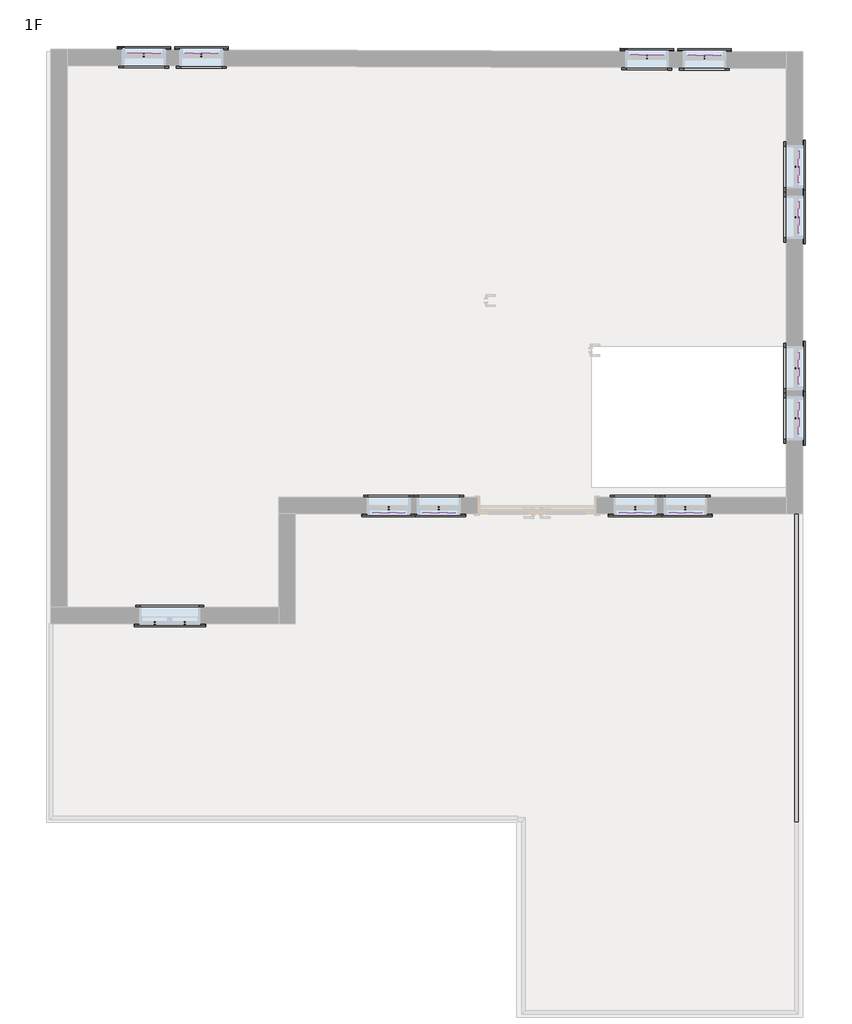
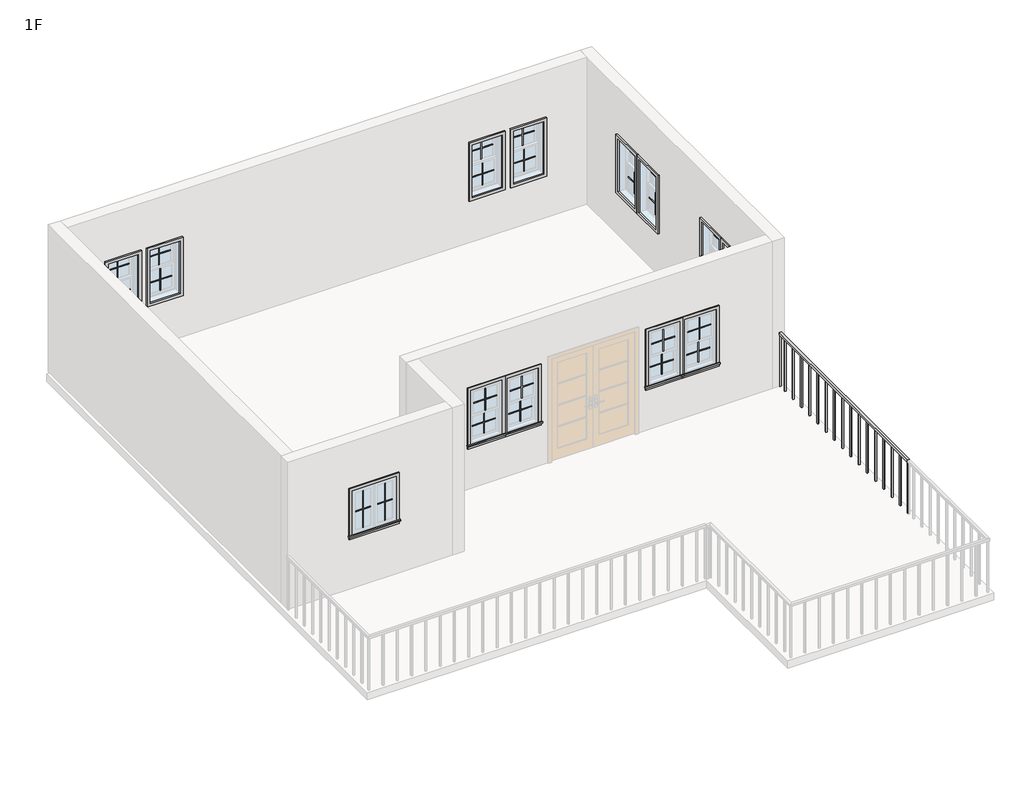
# One storey, part 2 of 2: 52 proxies, 1 railing.
"""IFC4 building model written with IfcOpenShell, lengths in millimetres."""

import ifcopenshell
import ifcopenshell.guid

model = None  # the IFC model being written
_history = None  # IfcOwnerHistory: only IFC2X3 demands one
_inside = {}  # id of a spatial element -> (the spatial element, [elements in it])
_under = {}  # id of a project, library or spatial element -> (it, [spatial elements below it])
_declared = {}  # id of a project -> (the project, [libraries it declares])
_typed = {}  # id of a type object -> (the type object, [elements of that type])
_made_of = {}  # id of a material, layer set ... -> (it, [elements and type objects made of it])


def new_model(schema):
    """Start an empty IFC model of exactly this schema.

    Asked for "IFC4X3", IfcOpenShell would pick the latest addendum, in which some entities
    have other attributes; the version numbers below select the first issue.
    IFC2X3 requires an IfcOwnerHistory on every rooted entity: one is made here for all.
    """
    global model, _history
    if schema == "IFC4X3":
        model = ifcopenshell.file(schema_version=(4, 3, 0, 0))
    else:
        model = ifcopenshell.file(schema=schema)
    _inside.clear()
    _under.clear()
    _declared.clear()
    _typed.clear()
    _made_of.clear()
    _history = None
    if model.schema == "IFC2X3":
        org = make("IfcOrganization", Name="unknown")
        user = make(
            "IfcPersonAndOrganization",
            ThePerson=make("IfcPerson", FamilyName="unknown"),
            TheOrganization=org,
        )
        app = make(
            "IfcApplication",
            ApplicationDeveloper=org,
            Version="unknown",
            ApplicationFullName="unknown",
            ApplicationIdentifier="unknown",
        )
        _history = make(
            "IfcOwnerHistory",
            OwningUser=user,
            OwningApplication=app,
            ChangeAction="ADDED",
            CreationDate=0,
        )
    return model


def make(cls, **values):
    """One entity of the class cls with the attributes given. An attribute that is None is left unset."""
    return model.create_entity(
        cls, **{name: value for name, value in values.items() if value is not None}
    )


def rooted(cls, **values):
    """An entity with a GlobalId (a new one), such as an element, a storey or a relation."""
    return make(cls, GlobalId=ifcopenshell.guid.new(), OwnerHistory=_history, **values)


def si_unit(unit_type, name, prefix=None):
    """IfcSIUnit, for example si_unit("LENGTHUNIT", "METRE", prefix="MILLI")."""
    return make("IfcSIUnit", UnitType=unit_type, Prefix=prefix, Name=name)


def assignment(units):
    """IfcUnitAssignment: the units of a project."""
    return None if units is None else make("IfcUnitAssignment", Units=units)


def point(xyz):
    """IfcCartesianPoint."""
    return None if xyz is None else make("IfcCartesianPoint", Coordinates=xyz)


def direction(xyz):
    """IfcDirection."""
    return None if xyz is None else make("IfcDirection", DirectionRatios=xyz)


def frame(location, z_axis=None, x_axis=None):
    """IfcAxis2Placement3D, a coordinate frame: its origin and axes. An axis left out is left unset."""
    return make(
        "IfcAxis2Placement3D",
        Location=point(location),
        Axis=direction(z_axis),
        RefDirection=direction(x_axis),
    )


def origin():
    """The frame at (0, 0, 0) with its axes left unset."""
    return frame((0.0, 0.0, 0.0))


def origin_with_axes():
    """The frame at (0, 0, 0) with the z axis (0, 0, 1) and the x axis (1, 0, 0) written out."""
    return frame((0.0, 0.0, 0.0), z_axis=(0.0, 0.0, 1.0), x_axis=(1.0, 0.0, 0.0))


def place(relative_to, where):
    """IfcLocalPlacement: puts the frame where relative to a parent placement (None: the world)."""
    return make(
        "IfcLocalPlacement", PlacementRelTo=relative_to, RelativePlacement=where
    )


def context(
    kind, dimensions, precision=None, world=None, true_north=None, identifier=None
):
    """IfcGeometricRepresentationContext, for example the 3D "Model" context."""
    return make(
        "IfcGeometricRepresentationContext",
        ContextIdentifier=identifier,
        ContextType=kind,
        CoordinateSpaceDimension=dimensions,
        Precision=precision,
        WorldCoordinateSystem=world,
        TrueNorth=true_north,
    )


def project(units=None, contexts=None):
    """IfcProject with its units and contexts."""
    return rooted(
        "IfcProject",
        Name="project",
        RepresentationContexts=contexts,
        UnitsInContext=assignment(units),
    )


def spatial(cls, under=None, at=None, **own):
    """A site, building, storey or space (cls), placed at a placement, below another one or the project."""
    s = rooted(cls, ObjectPlacement=at, **own)
    if under is not None:
        _under.setdefault(under.id(), (under, []))[1].append(s)
    return s


def polyline(points):
    """IfcPolyline through the points."""
    return make("IfcPolyline", Points=[point(p) for p in points])


def outline(outer, holes=None, kind="AREA"):
    """IfcArbitraryClosedProfileDef: a profile drawn as a closed curve; with holes, ...WithVoids."""
    if holes is None:
        return make("IfcArbitraryClosedProfileDef", ProfileType=kind, OuterCurve=outer)
    return make(
        "IfcArbitraryProfileDefWithVoids",
        ProfileType=kind,
        OuterCurve=outer,
        InnerCurves=holes,
    )


def extrude(swept, where, along, depth):
    """IfcExtrudedAreaSolid: the profile swept, set in the frame where, extruded along a direction by depth."""
    return make(
        "IfcExtrudedAreaSolid",
        SweptArea=swept,
        Position=where,
        ExtrudedDirection=direction(along),
        Depth=depth,
    )


def shape(context_of_items, identifier, shape_type, items):
    """IfcShapeRepresentation: the items that make up one representation, for example the "Body"."""
    return make(
        "IfcShapeRepresentation",
        ContextOfItems=context_of_items,
        RepresentationIdentifier=identifier,
        RepresentationType=shape_type,
        Items=items,
    )


def source(mapping_origin, context_of_items, identifier, shape_type, items):
    """IfcRepresentationMap: a shape defined once, which mapped items show again and again."""
    return make(
        "IfcRepresentationMap",
        MappingOrigin=mapping_origin,
        MappedRepresentation=shape(context_of_items, identifier, shape_type, items),
    )


def transform(
    local_origin,
    x_axis=None,
    y_axis=None,
    z_axis=None,
    scale=None,
    scale2=None,
    scale3=None,
    uniform=True,
):
    """IfcCartesianTransformationOperator3D, or its non-uniform kind. x_axis, y_axis, z_axis: its Axis1, 2, 3."""
    if uniform:
        return make(
            "IfcCartesianTransformationOperator3D",
            Axis1=direction(x_axis),
            Axis2=direction(y_axis),
            LocalOrigin=point(local_origin),
            Scale=scale,
            Axis3=direction(z_axis),
        )
    return make(
        "IfcCartesianTransformationOperator3DnonUniform",
        Axis1=direction(x_axis),
        Axis2=direction(y_axis),
        LocalOrigin=point(local_origin),
        Scale=scale,
        Axis3=direction(z_axis),
        Scale2=scale2,
        Scale3=scale3,
    )


def mapped(mapping_source, mapping_target):
    """IfcMappedItem: shows the shape of a source again, moved by a transform."""
    return make(
        "IfcMappedItem", MappingSource=mapping_source, MappingTarget=mapping_target
    )


def made_of(thing, what):
    """Note that an element or type object is made of a material, layer set ...; save() writes the relation."""
    if what is not None:
        _made_of.setdefault(what.id(), (what, []))[1].append(thing)
    return thing


def element(
    cls,
    number,
    at=None,
    inside=None,
    cuts=None,
    type_object=None,
    material=None,
    context=None,
    identifier="Body",
    shape_type=None,
    held_by="IfcProductDefinitionShape",
    body=None,
    shapes=None,
    **own,
):
    """One element of the class cls, such as IfcWall. Its Tag is "e" and its number.

    at: its placement. inside: the storey or other place that contains it. cuts: it is an
    opening in that element (IfcRelVoidsElement). A single representation is given by context,
    identifier, shape_type and body (its items); several are given by shapes. held_by: the class
    of the entity that holds the representations. save() writes the other relations.
    """
    e = rooted(cls, Tag="e%d" % number, ObjectPlacement=at, **own)
    if body is not None:
        shapes = [shape(context, identifier, shape_type, body)]
    if shapes is not None:
        e.Representation = make(held_by, Representations=shapes)
    if inside is not None:
        _inside.setdefault(inside.id(), (inside, []))[1].append(e)
    if cuts is not None:
        rooted(
            "IfcRelVoidsElement", RelatingBuildingElement=cuts, RelatedOpeningElement=e
        )
    if type_object is not None:
        _typed.setdefault(type_object.id(), (type_object, []))[1].append(e)
    return made_of(e, material)


def aggregate(whole, parts):
    """IfcRelAggregates: a whole, such as a stair, and the parts it consists of."""
    return rooted("IfcRelAggregates", RelatingObject=whole, RelatedObjects=parts)


def save(model, path):
    """Write the relations noted so far, then the file.

    IfcRelAggregates (storeys below a building ...), IfcRelContainedInSpatialStructure (elements
    in a storey), IfcRelDefinesByType, IfcRelAssociatesMaterial and IfcRelDeclares: one each for
    every whole, place, type object, material and project.
    """
    for whole, parts in _under.values():
        aggregate(whole, parts)
    for where, things in _inside.values():
        rooted(
            "IfcRelContainedInSpatialStructure",
            RelatedElements=things,
            RelatingStructure=where,
        )
    for kind, things in _typed.values():
        rooted("IfcRelDefinesByType", RelatedObjects=things, RelatingType=kind)
    for what, things in _made_of.values():
        rooted("IfcRelAssociatesMaterial", RelatedObjects=things, RelatingMaterial=what)
    for by, libraries in _declared.values():
        rooted("IfcRelDeclares", RelatingContext=by, RelatedDefinitions=libraries)
    model.write(path)


def m_muntin_pattern_2x2_m_muntin_pattern_2x2_62480ac4(model_context):
    return source(origin(), model_context, "Body", "SweptSolid", [
        extrude(outline(polyline([(386.5, -6.35), (386.5, -144.2375), (373.8, -144.2375), (373.8, -6.35), (0.0, -6.35), (0.0, 6.35), (373.8, 6.35), (373.8, 144.2375), (386.5, 144.2375), (386.5, 6.35), (760.3, 6.35), (760.3, -6.35), (386.5, -6.35)])), frame((0.0, 9.525, 0.0), z_axis=(0.0, 1.0, 0.0), x_axis=(0.0, 0.0, 1.0)), (0.0, 0.0, 1.0), 12.7),
        extrude(outline(polyline([(386.5, -6.35), (386.5, -144.2375), (373.8, -144.2375), (373.8, -6.35), (0.0, -6.35), (0.0, 6.35), (373.8, 6.35), (373.8, 144.2375), (386.5, 144.2375), (386.5, 6.35), (760.3, 6.35), (760.3, -6.35), (386.5, -6.35)])), frame((0.0, -22.225, 0.0), z_axis=(0.0, 1.0, 0.0), x_axis=(0.0, 0.0, 1.0)), (0.0, 0.0, 1.0), 12.7),
    ])


def m_muntin_pattern_2x2_m_muntin_pattern_2x2_4fd78f17(model_context):
    return source(origin(), model_context, "Body", "SweptSolid", [
        extrude(outline(polyline([(386.5, -6.35), (386.5, -144.2375), (373.8, -144.2375), (373.8, -6.35), (0.0, -6.35), (0.0, 6.35), (373.8, 6.35), (373.8, 144.2375), (386.5, 144.2375), (386.5, 6.35), (760.3, 6.35), (760.3, -6.35), (386.5, -6.35)])), frame((0.0, -22.225, 0.0), z_axis=(0.0, 1.0, 0.0), x_axis=(0.0, 0.0, 1.0)), (0.0, 0.0, 1.0), 12.7),
        extrude(outline(polyline([(386.5, -6.35), (386.5, -144.2375), (373.8, -144.2375), (373.8, -6.35), (0.0, -6.35), (0.0, 6.35), (373.8, 6.35), (373.8, 144.2375), (386.5, 144.2375), (386.5, 6.35), (760.3, 6.35), (760.3, -6.35), (386.5, -6.35)])), frame((0.0, 9.525, 0.0), z_axis=(0.0, 1.0, 0.0), x_axis=(0.0, 0.0, 1.0)), (0.0, 0.0, 1.0), 12.7),
    ])


def m_muntin_pattern_2x2_m_muntin_pattern_2x2_6483b455(model_context):
    return source(origin(), model_context, "Body", "SweptSolid", [
        extrude(outline(polyline([(232.1375, -6.35), (232.1375, -223.8), (219.4375, -223.8), (219.4375, -6.35), (0.0, -6.35), (0.0, 6.35), (219.4375, 6.35), (219.4375, 223.8), (232.1375, 223.8), (232.1375, 6.35), (451.575, 6.35), (451.575, -6.35), (232.1375, -6.35)])), frame((0.0, 9.525, 0.0), z_axis=(0.0, 1.0, 0.0), x_axis=(0.0, 0.0, 1.0)), (0.0, 0.0, 1.0), 12.7),
        extrude(outline(polyline([(232.1375, -6.35), (232.1375, -223.8), (219.4375, -223.8), (219.4375, -6.35), (0.0, -6.35), (0.0, 6.35), (219.4375, 6.35), (219.4375, 223.8), (232.1375, 223.8), (232.1375, 6.35), (451.575, 6.35), (451.575, -6.35), (232.1375, -6.35)])), frame((0.0, -22.225, 0.0), z_axis=(0.0, 1.0, 0.0), x_axis=(0.0, 0.0, 1.0)), (0.0, 0.0, 1.0), 12.7),
    ])


def m_trim_window_exterior_flat_with_sill_90d3a428(model_context):
    return source(origin(), model_context, "Body", "SweptSolid", [
        extrude(outline(polyline([(485.0, -920.4323709), (485.0, -980.4323709), (-485.0, -980.4323709), (-485.0, -920.4323709), (485.0, -920.4323709)])), origin_with_axes(), (0.0, 0.0, 1.0), 19.05),
        extrude(outline(polyline([(-930.0, 38.1), (-902.4580645, 38.1), (-900.0, 19.05), (-900.0, 0.0), (-920.4323709, 0.0), (-920.4323709, 19.05), (-930.0, 19.05), (-930.0, 38.1)])), frame((-497.7, 0.0, 0.0), z_axis=(1.0, 0.0, 0.0), x_axis=(0.0, 1.0, 0.0)), (0.0, 0.0, 1.0), 995.4),
        extrude(outline(polyline([(-485.0, 60.0), (485.0, 60.0), (485.0, -900.0), (425.0, -900.0), (425.0, 0.0), (-425.0, 0.0), (-425.0, -900.0), (-485.0, -900.0), (-485.0, 60.0)])), origin_with_axes(), (0.0, 0.0, 1.0), 19.05),
    ])


def m_trim_window_exterior_flat_with_sill_4c9fee41(model_context):
    return source(origin(), model_context, "Body", "SweptSolid", [
        extrude(outline(polyline([(360.0, -1120.4323709), (360.0, -1180.4323709), (-360.0, -1180.4323709), (-360.0, -1120.4323709), (360.0, -1120.4323709)])), origin_with_axes(), (0.0, 0.0, 1.0), 19.05),
        extrude(outline(polyline([(-1130.0, 38.1), (-1102.4580645, 38.1), (-1100.0, 19.05), (-1100.0, 0.0), (-1120.4323709, 0.0), (-1120.4323709, 19.05), (-1130.0, 19.05), (-1130.0, 38.1)])), frame((-372.7, 0.0, 0.0), z_axis=(1.0, 0.0, 0.0), x_axis=(0.0, 1.0, 0.0)), (0.0, 0.0, 1.0), 745.4),
        extrude(outline(polyline([(-360.0, 60.0), (360.0, 60.0), (360.0, -1100.0), (300.0, -1100.0), (300.0, 0.0), (-300.0, 0.0), (-300.0, -1100.0), (-360.0, -1100.0), (-360.0, 60.0)])), origin_with_axes(), (0.0, 0.0, 1.0), 19.05),
    ])


def m_trim_window_interior_flat_picture_frame_6ca9b1f8(model_context):
    return source(origin(), model_context, "Body", "SweptSolid", [
        extrude(outline(polyline([(472.3, 47.3), (472.3, -947.3), (-472.3, -947.3), (-472.3, 47.3), (472.3, 47.3)]), holes=[polyline([(412.3, -12.7), (-412.3, -12.7), (-412.3, -887.3), (412.3, -887.3), (412.3, -12.7)])]), origin_with_axes(), (0.0, 0.0, 1.0), 30.0),
    ])


def m_trim_window_interior_flat_picture_frame_87adca9b(model_context):
    return source(origin(), model_context, "Body", "SweptSolid", [
        extrude(outline(polyline([(347.3, 47.3), (347.3, -1147.3), (-347.3, -1147.3), (-347.3, 47.3), (347.3, 47.3)]), holes=[polyline([(287.3, -12.7), (-287.3, -12.7), (-287.3, -1087.3), (287.3, -1087.3), (287.3, -12.7)])]), origin_with_axes(), (0.0, 0.0, 1.0), 30.0),
    ])


model = new_model("IFC4")

# Units and contexts
model_context = context("Model", 3, world=origin())
ifc_project = project(units=[si_unit("LENGTHUNIT", "METRE", prefix="MILLI")], contexts=[model_context])

# Site, building, storey
site = spatial("IfcSite", under=ifc_project)
building = spatial("IfcBuilding", under=site)
storey = spatial("IfcBuildingStorey", under=building, Name="1F", Elevation=3450.0)

# Proxies
placement = place(None, origin())
m_muntin_pattern_2x2_m_muntin_pattern_2x2_shape = m_muntin_pattern_2x2_m_muntin_pattern_2x2_62480ac4(model_context)
element("IfcBuildingElementProxy", 1, Name="M_Muntin Pattern_2x2 : M_Muntin Pattern_2x2", ObjectType="M_Muntin Pattern_2x2 : M_Muntin Pattern_2x2", at=placement, inside=storey, context=model_context, shape_type="MappedRepresentation", body=[
    mapped(m_muntin_pattern_2x2_m_muntin_pattern_2x2_shape, transform((-17210.6778863, -85.4683886, 4624.9759098), x_axis=(-1.0, 0.0, 0.0), y_axis=(0.0, -1.0, 0.0), z_axis=(0.0, 0.0, 1.0))),
])
m_muntin_pattern_2x2_m_muntin_pattern_2x2_2_shape = m_muntin_pattern_2x2_m_muntin_pattern_2x2_4fd78f17(model_context)
element("IfcBuildingElementProxy", 2, Name="M_Muntin Pattern_2x2 : M_Muntin Pattern_2x2", ObjectType="M_Muntin Pattern_2x2 : M_Muntin Pattern_2x2", at=placement, inside=storey, context=model_context, shape_type="MappedRepresentation", body=[
    mapped(m_muntin_pattern_2x2_m_muntin_pattern_2x2_2_shape, transform((-17632.5028863, -85.4683886, 4624.9759098), x_axis=(1.0, 0.0, 0.0), y_axis=(0.0, 1.0, 0.0), z_axis=(0.0, 0.0, 1.0))),
])
m_muntin_pattern_2x2_m_muntin_pattern_2x2_3_shape = m_muntin_pattern_2x2_m_muntin_pattern_2x2_6483b455(model_context)
element("IfcBuildingElementProxy", 3, Name="M_Muntin Pattern_2x2 : M_Muntin Pattern_2x2", ObjectType="M_Muntin Pattern_2x2 : M_Muntin Pattern_2x2", at=placement, inside=storey, context=model_context, shape_type="MappedRepresentation", body=[
    mapped(m_muntin_pattern_2x2_m_muntin_pattern_2x2_3_shape, transform((-14376.5903863, 1469.9316114, 4936.625), x_axis=(-1.0, 0.0, 0.0), y_axis=(0.0, -1.0, 0.0), z_axis=(0.0, 0.0, 1.0))),
])
element("IfcBuildingElementProxy", 4, Name="M_Muntin Pattern_2x2 : M_Muntin Pattern_2x2", ObjectType="M_Muntin Pattern_2x2 : M_Muntin Pattern_2x2", at=placement, inside=storey, context=model_context, shape_type="MappedRepresentation", body=[
    mapped(m_muntin_pattern_2x2_m_muntin_pattern_2x2_3_shape, transform((-14376.5903863, 1514.3816114, 4440.6), x_axis=(-1.0, 0.0, 0.0), y_axis=(0.0, -1.0, 0.0), z_axis=(0.0, 0.0, 1.0))),
])
element("IfcBuildingElementProxy", 5, Name="M_Muntin Pattern_2x2 : M_Muntin Pattern_2x2", ObjectType="M_Muntin Pattern_2x2 : M_Muntin Pattern_2x2", at=placement, inside=storey, context=model_context, shape_type="MappedRepresentation", body=[
    mapped(m_muntin_pattern_2x2_m_muntin_pattern_2x2_3_shape, transform((-13676.5903863, 1469.9316114, 4936.625), x_axis=(-1.0, 0.0, 0.0), y_axis=(0.0, -1.0, 0.0), z_axis=(0.0, 0.0, 1.0))),
])
element("IfcBuildingElementProxy", 6, Name="M_Muntin Pattern_2x2 : M_Muntin Pattern_2x2", ObjectType="M_Muntin Pattern_2x2 : M_Muntin Pattern_2x2", at=placement, inside=storey, context=model_context, shape_type="MappedRepresentation", body=[
    mapped(m_muntin_pattern_2x2_m_muntin_pattern_2x2_3_shape, transform((-13676.5903863, 1514.3816114, 4440.6), x_axis=(-1.0, 0.0, 0.0), y_axis=(0.0, -1.0, 0.0), z_axis=(0.0, 0.0, 1.0))),
])
element("IfcBuildingElementProxy", 7, Name="M_Muntin Pattern_2x2 : M_Muntin Pattern_2x2", ObjectType="M_Muntin Pattern_2x2 : M_Muntin Pattern_2x2", at=placement, inside=storey, context=model_context, shape_type="MappedRepresentation", body=[
    mapped(m_muntin_pattern_2x2_m_muntin_pattern_2x2_3_shape, transform((-10946.5903863, 1469.9316114, 4936.625), x_axis=(-1.0, 0.0, 0.0), y_axis=(0.0, -1.0, 0.0), z_axis=(0.0, 0.0, 1.0))),
])
element("IfcBuildingElementProxy", 8, Name="M_Muntin Pattern_2x2 : M_Muntin Pattern_2x2", ObjectType="M_Muntin Pattern_2x2 : M_Muntin Pattern_2x2", at=placement, inside=storey, context=model_context, shape_type="MappedRepresentation", body=[
    mapped(m_muntin_pattern_2x2_m_muntin_pattern_2x2_3_shape, transform((-10946.5903863, 1514.3816114, 4440.6), x_axis=(-1.0, 0.0, 0.0), y_axis=(0.0, -1.0, 0.0), z_axis=(0.0, 0.0, 1.0))),
])
element("IfcBuildingElementProxy", 9, Name="M_Muntin Pattern_2x2 : M_Muntin Pattern_2x2", ObjectType="M_Muntin Pattern_2x2 : M_Muntin Pattern_2x2", at=placement, inside=storey, context=model_context, shape_type="MappedRepresentation", body=[
    mapped(m_muntin_pattern_2x2_m_muntin_pattern_2x2_3_shape, transform((-10246.5903863, 1469.9316114, 4936.625), x_axis=(-1.0, 0.0, 0.0), y_axis=(0.0, -1.0, 0.0), z_axis=(0.0, 0.0, 1.0))),
])
element("IfcBuildingElementProxy", 10, Name="M_Muntin Pattern_2x2 : M_Muntin Pattern_2x2", ObjectType="M_Muntin Pattern_2x2 : M_Muntin Pattern_2x2", at=placement, inside=storey, context=model_context, shape_type="MappedRepresentation", body=[
    mapped(m_muntin_pattern_2x2_m_muntin_pattern_2x2_3_shape, transform((-10246.5903863, 1514.3816114, 4440.6), x_axis=(-1.0, 0.0, 0.0), y_axis=(0.0, -1.0, 0.0), z_axis=(0.0, 0.0, 1.0))),
])
element("IfcBuildingElementProxy", 11, Name="M_Muntin Pattern_2x2 : M_Muntin Pattern_2x2", ObjectType="M_Muntin Pattern_2x2 : M_Muntin Pattern_2x2", at=placement, inside=storey, context=model_context, shape_type="MappedRepresentation", body=[
    mapped(m_muntin_pattern_2x2_m_muntin_pattern_2x2_3_shape, transform((-8651.5153863, 2765.0066114, 4936.625), x_axis=(0.0, -1.0, 0.0), y_axis=(1.0, 0.0, 0.0), z_axis=(0.0, 0.0, 1.0))),
])
element("IfcBuildingElementProxy", 12, Name="M_Muntin Pattern_2x2 : M_Muntin Pattern_2x2", ObjectType="M_Muntin Pattern_2x2 : M_Muntin Pattern_2x2", at=placement, inside=storey, context=model_context, shape_type="MappedRepresentation", body=[
    mapped(m_muntin_pattern_2x2_m_muntin_pattern_2x2_3_shape, transform((-8695.9653863, 2765.0066114, 4440.6), x_axis=(0.0, -1.0, 0.0), y_axis=(1.0, 0.0, 0.0), z_axis=(0.0, 0.0, 1.0))),
])
element("IfcBuildingElementProxy", 13, Name="M_Muntin Pattern_2x2 : M_Muntin Pattern_2x2", ObjectType="M_Muntin Pattern_2x2 : M_Muntin Pattern_2x2", at=placement, inside=storey, context=model_context, shape_type="MappedRepresentation", body=[
    mapped(m_muntin_pattern_2x2_m_muntin_pattern_2x2_3_shape, transform((-8651.5153863, 3465.0066114, 4936.625), x_axis=(0.0, -1.0, 0.0), y_axis=(1.0, 0.0, 0.0), z_axis=(0.0, 0.0, 1.0))),
])
element("IfcBuildingElementProxy", 14, Name="M_Muntin Pattern_2x2 : M_Muntin Pattern_2x2", ObjectType="M_Muntin Pattern_2x2 : M_Muntin Pattern_2x2", at=placement, inside=storey, context=model_context, shape_type="MappedRepresentation", body=[
    mapped(m_muntin_pattern_2x2_m_muntin_pattern_2x2_3_shape, transform((-8695.9653863, 3465.0066114, 4440.6), x_axis=(0.0, -1.0, 0.0), y_axis=(1.0, 0.0, 0.0), z_axis=(0.0, 0.0, 1.0))),
])
element("IfcBuildingElementProxy", 15, Name="M_Muntin Pattern_2x2 : M_Muntin Pattern_2x2", ObjectType="M_Muntin Pattern_2x2 : M_Muntin Pattern_2x2", at=placement, inside=storey, context=model_context, shape_type="MappedRepresentation", body=[
    mapped(m_muntin_pattern_2x2_m_muntin_pattern_2x2_3_shape, transform((-8651.5153863, 5565.0066114, 4936.625), x_axis=(0.0, -1.0, 0.0), y_axis=(1.0, 0.0, 0.0), z_axis=(0.0, 0.0, 1.0))),
])
element("IfcBuildingElementProxy", 16, Name="M_Muntin Pattern_2x2 : M_Muntin Pattern_2x2", ObjectType="M_Muntin Pattern_2x2 : M_Muntin Pattern_2x2", at=placement, inside=storey, context=model_context, shape_type="MappedRepresentation", body=[
    mapped(m_muntin_pattern_2x2_m_muntin_pattern_2x2_3_shape, transform((-8695.9653863, 5565.0066114, 4440.6), x_axis=(0.0, -1.0, 0.0), y_axis=(1.0, 0.0, 0.0), z_axis=(0.0, 0.0, 1.0))),
])
element("IfcBuildingElementProxy", 17, Name="M_Muntin Pattern_2x2 : M_Muntin Pattern_2x2", ObjectType="M_Muntin Pattern_2x2 : M_Muntin Pattern_2x2", at=placement, inside=storey, context=model_context, shape_type="MappedRepresentation", body=[
    mapped(m_muntin_pattern_2x2_m_muntin_pattern_2x2_3_shape, transform((-8651.5153863, 6265.0066114, 4936.625), x_axis=(0.0, -1.0, 0.0), y_axis=(1.0, 0.0, 0.0), z_axis=(0.0, 0.0, 1.0))),
])
element("IfcBuildingElementProxy", 18, Name="M_Muntin Pattern_2x2 : M_Muntin Pattern_2x2", ObjectType="M_Muntin Pattern_2x2 : M_Muntin Pattern_2x2", at=placement, inside=storey, context=model_context, shape_type="MappedRepresentation", body=[
    mapped(m_muntin_pattern_2x2_m_muntin_pattern_2x2_3_shape, transform((-8695.9653863, 6265.0066114, 4440.6), x_axis=(0.0, -1.0, 0.0), y_axis=(1.0, 0.0, 0.0), z_axis=(0.0, 0.0, 1.0))),
])
element("IfcBuildingElementProxy", 19, Name="M_Muntin Pattern_2x2 : M_Muntin Pattern_2x2", ObjectType="M_Muntin Pattern_2x2 : M_Muntin Pattern_2x2", at=placement, inside=storey, context=model_context, shape_type="MappedRepresentation", body=[
    mapped(m_muntin_pattern_2x2_m_muntin_pattern_2x2_3_shape, transform((-9981.2144778, 7835.2998038, 4936.625), x_axis=(0.9999926882412296, -0.0038240638173662514, 0.0), y_axis=(0.0038240638173662514, 0.9999926882412296, 0.0), z_axis=(0.0, 0.0, 1.0))),
])
element("IfcBuildingElementProxy", 20, Name="M_Muntin Pattern_2x2 : M_Muntin Pattern_2x2", ObjectType="M_Muntin Pattern_2x2 : M_Muntin Pattern_2x2", at=placement, inside=storey, context=model_context, shape_type="MappedRepresentation", body=[
    mapped(m_muntin_pattern_2x2_m_muntin_pattern_2x2_3_shape, transform((-9981.3844574, 7790.8501288, 4440.6), x_axis=(0.9999926882412296, -0.0038240638173662514, 0.0), y_axis=(0.0038240638173662514, 0.9999926882412296, 0.0), z_axis=(0.0, 0.0, 1.0))),
])
element("IfcBuildingElementProxy", 21, Name="M_Muntin Pattern_2x2 : M_Muntin Pattern_2x2", ObjectType="M_Muntin Pattern_2x2 : M_Muntin Pattern_2x2", at=placement, inside=storey, context=model_context, shape_type="MappedRepresentation", body=[
    mapped(m_muntin_pattern_2x2_m_muntin_pattern_2x2_3_shape, transform((-10781.2086284, 7838.3590548, 4936.625), x_axis=(0.9999926882412296, -0.0038240638173662514, 0.0), y_axis=(0.0038240638173662514, 0.9999926882412296, 0.0), z_axis=(0.0, 0.0, 1.0))),
])
element("IfcBuildingElementProxy", 22, Name="M_Muntin Pattern_2x2 : M_Muntin Pattern_2x2", ObjectType="M_Muntin Pattern_2x2 : M_Muntin Pattern_2x2", at=placement, inside=storey, context=model_context, shape_type="MappedRepresentation", body=[
    mapped(m_muntin_pattern_2x2_m_muntin_pattern_2x2_3_shape, transform((-10781.378608, 7793.9093798, 4440.6), x_axis=(0.9999926882412296, -0.0038240638173662514, 0.0), y_axis=(0.0038240638173662514, 0.9999926882412296, 0.0), z_axis=(0.0, 0.0, 1.0))),
])
element("IfcBuildingElementProxy", 23, Name="M_Muntin Pattern_2x2 : M_Muntin Pattern_2x2", ObjectType="M_Muntin Pattern_2x2 : M_Muntin Pattern_2x2", at=placement, inside=storey, context=model_context, shape_type="MappedRepresentation", body=[
    mapped(m_muntin_pattern_2x2_m_muntin_pattern_2x2_3_shape, transform((-17781.1574461, 7865.1275015, 4936.625), x_axis=(0.9999926882412296, -0.0038240638173662514, 0.0), y_axis=(0.0038240638173662514, 0.9999926882412296, 0.0), z_axis=(0.0, 0.0, 1.0))),
])
element("IfcBuildingElementProxy", 24, Name="M_Muntin Pattern_2x2 : M_Muntin Pattern_2x2", ObjectType="M_Muntin Pattern_2x2 : M_Muntin Pattern_2x2", at=placement, inside=storey, context=model_context, shape_type="MappedRepresentation", body=[
    mapped(m_muntin_pattern_2x2_m_muntin_pattern_2x2_3_shape, transform((-17781.3274257, 7820.6778265, 4440.6), x_axis=(0.9999926882412296, -0.0038240638173662514, 0.0), y_axis=(0.0038240638173662514, 0.9999926882412296, 0.0), z_axis=(0.0, 0.0, 1.0))),
])
element("IfcBuildingElementProxy", 25, Name="M_Muntin Pattern_2x2 : M_Muntin Pattern_2x2", ObjectType="M_Muntin Pattern_2x2 : M_Muntin Pattern_2x2", at=placement, inside=storey, context=model_context, shape_type="MappedRepresentation", body=[
    mapped(m_muntin_pattern_2x2_m_muntin_pattern_2x2_3_shape, transform((-16981.1632955, 7862.0682505, 4936.625), x_axis=(0.9999926882412296, -0.0038240638173662514, 0.0), y_axis=(0.0038240638173662514, 0.9999926882412296, 0.0), z_axis=(0.0, 0.0, 1.0))),
])
element("IfcBuildingElementProxy", 26, Name="M_Muntin Pattern_2x2 : M_Muntin Pattern_2x2", ObjectType="M_Muntin Pattern_2x2 : M_Muntin Pattern_2x2", at=placement, inside=storey, context=model_context, shape_type="MappedRepresentation", body=[
    mapped(m_muntin_pattern_2x2_m_muntin_pattern_2x2_3_shape, transform((-16981.3332751, 7817.6185755, 4440.6), x_axis=(0.9999926882412296, -0.0038240638173662514, 0.0), y_axis=(0.0038240638173662514, 0.9999926882412296, 0.0), z_axis=(0.0, 0.0, 1.0))),
])
m_trim_window_exterior_flat_with_sill_shape = m_trim_window_exterior_flat_with_sill_90d3a428(model_context)
element("IfcBuildingElementProxy", 27, Name="M_Trim-Window-Exterior-Flat : with Sill", ObjectType="M_Trim-Window-Exterior-Flat : with Sill", at=placement, inside=storey, context=model_context, shape_type="MappedRepresentation", body=[
    mapped(m_trim_window_exterior_flat_with_sill_shape, transform((-17421.5903863, -94.9933886, 5455.1259098), x_axis=(1.0, 0.0, 0.0), y_axis=(0.0, 0.0, 1.0), z_axis=(0.0, -1.0, 0.0))),
])
m_trim_window_exterior_flat_with_sill_2_shape = m_trim_window_exterior_flat_with_sill_4c9fee41(model_context)
element("IfcBuildingElementProxy", 28, Name="M_Trim-Window-Exterior-Flat : with Sill", ObjectType="M_Trim-Window-Exterior-Flat : with Sill", at=placement, inside=storey, context=model_context, shape_type="MappedRepresentation", body=[
    mapped(m_trim_window_exterior_flat_with_sill_2_shape, transform((-14376.5903863, 1435.0066114, 5464.4), x_axis=(1.0, 0.0, 0.0), y_axis=(0.0, 0.0, 1.0), z_axis=(0.0, -1.0, 0.0))),
])
element("IfcBuildingElementProxy", 29, Name="M_Trim-Window-Exterior-Flat : with Sill", ObjectType="M_Trim-Window-Exterior-Flat : with Sill", at=placement, inside=storey, context=model_context, shape_type="MappedRepresentation", body=[
    mapped(m_trim_window_exterior_flat_with_sill_2_shape, transform((-13676.5903863, 1435.0066114, 5464.4), x_axis=(1.0, 0.0, 0.0), y_axis=(0.0, 0.0, 1.0), z_axis=(0.0, -1.0, 0.0))),
])
element("IfcBuildingElementProxy", 30, Name="M_Trim-Window-Exterior-Flat : with Sill", ObjectType="M_Trim-Window-Exterior-Flat : with Sill", at=placement, inside=storey, context=model_context, shape_type="MappedRepresentation", body=[
    mapped(m_trim_window_exterior_flat_with_sill_2_shape, transform((-10946.5903863, 1435.0066114, 5464.4), x_axis=(1.0, 0.0, 0.0), y_axis=(0.0, 0.0, 1.0), z_axis=(0.0, -1.0, 0.0))),
])
element("IfcBuildingElementProxy", 31, Name="M_Trim-Window-Exterior-Flat : with Sill", ObjectType="M_Trim-Window-Exterior-Flat : with Sill", at=placement, inside=storey, context=model_context, shape_type="MappedRepresentation", body=[
    mapped(m_trim_window_exterior_flat_with_sill_2_shape, transform((-10246.5903863, 1435.0066114, 5464.4), x_axis=(1.0, 0.0, 0.0), y_axis=(0.0, 0.0, 1.0), z_axis=(0.0, -1.0, 0.0))),
])
element("IfcBuildingElementProxy", 32, Name="M_Trim-Window-Exterior-Flat : with Sill", ObjectType="M_Trim-Window-Exterior-Flat : with Sill", at=placement, inside=storey, context=model_context, shape_type="MappedRepresentation", body=[
    mapped(m_trim_window_exterior_flat_with_sill_2_shape, transform((-8616.5903863, 2765.0066114, 5464.4), x_axis=(0.0, 1.0, 0.0), y_axis=(0.0, 0.0, 1.0), z_axis=(1.0, 0.0, 0.0))),
])
element("IfcBuildingElementProxy", 33, Name="M_Trim-Window-Exterior-Flat : with Sill", ObjectType="M_Trim-Window-Exterior-Flat : with Sill", at=placement, inside=storey, context=model_context, shape_type="MappedRepresentation", body=[
    mapped(m_trim_window_exterior_flat_with_sill_2_shape, transform((-8616.5903863, 3465.0066114, 5464.4), x_axis=(0.0, 1.0, 0.0), y_axis=(0.0, 0.0, 1.0), z_axis=(1.0, 0.0, 0.0))),
])
element("IfcBuildingElementProxy", 34, Name="M_Trim-Window-Exterior-Flat : with Sill", ObjectType="M_Trim-Window-Exterior-Flat : with Sill", at=placement, inside=storey, context=model_context, shape_type="MappedRepresentation", body=[
    mapped(m_trim_window_exterior_flat_with_sill_2_shape, transform((-8616.5903863, 5565.0066114, 5464.4), x_axis=(0.0, 1.0, 0.0), y_axis=(0.0, 0.0, 1.0), z_axis=(1.0, 0.0, 0.0))),
])
element("IfcBuildingElementProxy", 35, Name="M_Trim-Window-Exterior-Flat : with Sill", ObjectType="M_Trim-Window-Exterior-Flat : with Sill", at=placement, inside=storey, context=model_context, shape_type="MappedRepresentation", body=[
    mapped(m_trim_window_exterior_flat_with_sill_2_shape, transform((-8616.5903863, 6265.0066114, 5464.4), x_axis=(0.0, 1.0, 0.0), y_axis=(0.0, 0.0, 1.0), z_axis=(1.0, 0.0, 0.0))),
])
element("IfcBuildingElementProxy", 36, Name="M_Trim-Window-Exterior-Flat : with Sill", ObjectType="M_Trim-Window-Exterior-Flat : with Sill", at=placement, inside=storey, context=model_context, shape_type="MappedRepresentation", body=[
    mapped(m_trim_window_exterior_flat_with_sill_2_shape, transform((-9981.0809224, 7870.2245484, 5464.4), x_axis=(-0.9999926882412296, 0.0038240638173662514, 0.0), y_axis=(0.0, 0.0, 1.0), z_axis=(0.0038240638173662514, 0.9999926882412296, 0.0))),
])
element("IfcBuildingElementProxy", 37, Name="M_Trim-Window-Exterior-Flat : with Sill", ObjectType="M_Trim-Window-Exterior-Flat : with Sill", at=placement, inside=storey, context=model_context, shape_type="MappedRepresentation", body=[
    mapped(m_trim_window_exterior_flat_with_sill_2_shape, transform((-10781.0750729, 7873.2837994, 5464.4), x_axis=(-0.9999926882412296, 0.0038240638173662514, 0.0), y_axis=(0.0, 0.0, 1.0), z_axis=(0.0038240638173662514, 0.9999926882412296, 0.0))),
])
element("IfcBuildingElementProxy", 38, Name="M_Trim-Window-Exterior-Flat : with Sill", ObjectType="M_Trim-Window-Exterior-Flat : with Sill", at=placement, inside=storey, context=model_context, shape_type="MappedRepresentation", body=[
    mapped(m_trim_window_exterior_flat_with_sill_2_shape, transform((-17781.0238906, 7900.0522462, 5464.4), x_axis=(-0.9999926882412296, 0.0038240638173662514, 0.0), y_axis=(0.0, 0.0, 1.0), z_axis=(0.0038240638173662514, 0.9999926882412296, 0.0))),
])
element("IfcBuildingElementProxy", 39, Name="M_Trim-Window-Exterior-Flat : with Sill", ObjectType="M_Trim-Window-Exterior-Flat : with Sill", at=placement, inside=storey, context=model_context, shape_type="MappedRepresentation", body=[
    mapped(m_trim_window_exterior_flat_with_sill_2_shape, transform((-16981.02974, 7896.9929951, 5464.4), x_axis=(-0.9999926882412296, 0.0038240638173662514, 0.0), y_axis=(0.0, 0.0, 1.0), z_axis=(0.0038240638173662514, 0.9999926882412296, 0.0))),
])
m_trim_window_interior_flat_picture_frame_shape = m_trim_window_interior_flat_picture_frame_6ca9b1f8(model_context)
element("IfcBuildingElementProxy", 40, Name="M_Trim-Window-Interior-Flat : Picture Frame", ObjectType="M_Trim-Window-Interior-Flat : Picture Frame", at=placement, inside=storey, context=model_context, shape_type="MappedRepresentation", body=[
    mapped(m_trim_window_interior_flat_picture_frame_shape, transform((-17421.5903863, 135.0066114, 5455.1259098), x_axis=(-1.0, 0.0, 0.0), y_axis=(0.0, 0.0, 1.0), z_axis=(0.0, 1.0, 0.0))),
])
m_trim_window_interior_flat_picture_frame_2_shape = m_trim_window_interior_flat_picture_frame_87adca9b(model_context)
element("IfcBuildingElementProxy", 41, Name="M_Trim-Window-Interior-Flat : Picture Frame", ObjectType="M_Trim-Window-Interior-Flat : Picture Frame", at=placement, inside=storey, context=model_context, shape_type="MappedRepresentation", body=[
    mapped(m_trim_window_interior_flat_picture_frame_2_shape, transform((-14376.5903863, 1665.0066114, 5464.4), x_axis=(-1.0, 0.0, 0.0), y_axis=(0.0, 0.0, 1.0), z_axis=(0.0, 1.0, 0.0))),
])
element("IfcBuildingElementProxy", 42, Name="M_Trim-Window-Interior-Flat : Picture Frame", ObjectType="M_Trim-Window-Interior-Flat : Picture Frame", at=placement, inside=storey, context=model_context, shape_type="MappedRepresentation", body=[
    mapped(m_trim_window_interior_flat_picture_frame_2_shape, transform((-13676.5903863, 1665.0066114, 5464.4), x_axis=(-1.0, 0.0, 0.0), y_axis=(0.0, 0.0, 1.0), z_axis=(0.0, 1.0, 0.0))),
])
element("IfcBuildingElementProxy", 43, Name="M_Trim-Window-Interior-Flat : Picture Frame", ObjectType="M_Trim-Window-Interior-Flat : Picture Frame", at=placement, inside=storey, context=model_context, shape_type="MappedRepresentation", body=[
    mapped(m_trim_window_interior_flat_picture_frame_2_shape, transform((-10946.5903863, 1665.0066114, 5464.4), x_axis=(-1.0, 0.0, 0.0), y_axis=(0.0, 0.0, 1.0), z_axis=(0.0, 1.0, 0.0))),
])
element("IfcBuildingElementProxy", 44, Name="M_Trim-Window-Interior-Flat : Picture Frame", ObjectType="M_Trim-Window-Interior-Flat : Picture Frame", at=placement, inside=storey, context=model_context, shape_type="MappedRepresentation", body=[
    mapped(m_trim_window_interior_flat_picture_frame_2_shape, transform((-10246.5903863, 1665.0066114, 5464.4), x_axis=(-1.0, 0.0, 0.0), y_axis=(0.0, 0.0, 1.0), z_axis=(0.0, 1.0, 0.0))),
])
element("IfcBuildingElementProxy", 45, Name="M_Trim-Window-Interior-Flat : Picture Frame", ObjectType="M_Trim-Window-Interior-Flat : Picture Frame", at=placement, inside=storey, context=model_context, shape_type="MappedRepresentation", body=[
    mapped(m_trim_window_interior_flat_picture_frame_2_shape, transform((-8846.5903863, 2765.0066114, 5464.4), x_axis=(0.0, -1.0, 0.0), y_axis=(0.0, 0.0, 1.0), z_axis=(-1.0, 0.0, 0.0))),
])
element("IfcBuildingElementProxy", 46, Name="M_Trim-Window-Interior-Flat : Picture Frame", ObjectType="M_Trim-Window-Interior-Flat : Picture Frame", at=placement, inside=storey, context=model_context, shape_type="MappedRepresentation", body=[
    mapped(m_trim_window_interior_flat_picture_frame_2_shape, transform((-8846.5903863, 3465.0066114, 5464.4), x_axis=(0.0, -1.0, 0.0), y_axis=(0.0, 0.0, 1.0), z_axis=(-1.0, 0.0, 0.0))),
])
element("IfcBuildingElementProxy", 47, Name="M_Trim-Window-Interior-Flat : Picture Frame", ObjectType="M_Trim-Window-Interior-Flat : Picture Frame", at=placement, inside=storey, context=model_context, shape_type="MappedRepresentation", body=[
    mapped(m_trim_window_interior_flat_picture_frame_2_shape, transform((-8846.5903863, 5565.0066114, 5464.4), x_axis=(0.0, -1.0, 0.0), y_axis=(0.0, 0.0, 1.0), z_axis=(-1.0, 0.0, 0.0))),
])
element("IfcBuildingElementProxy", 48, Name="M_Trim-Window-Interior-Flat : Picture Frame", ObjectType="M_Trim-Window-Interior-Flat : Picture Frame", at=placement, inside=storey, context=model_context, shape_type="MappedRepresentation", body=[
    mapped(m_trim_window_interior_flat_picture_frame_2_shape, transform((-8846.5903863, 6265.0066114, 5464.4), x_axis=(0.0, -1.0, 0.0), y_axis=(0.0, 0.0, 1.0), z_axis=(-1.0, 0.0, 0.0))),
])
element("IfcBuildingElementProxy", 49, Name="M_Trim-Window-Interior-Flat : Picture Frame", ObjectType="M_Trim-Window-Interior-Flat : Picture Frame", at=placement, inside=storey, context=model_context, shape_type="MappedRepresentation", body=[
    mapped(m_trim_window_interior_flat_picture_frame_2_shape, transform((-9981.960457, 7640.2262301, 5464.4), x_axis=(0.9999926882412296, -0.0038240638173662514, 0.0), y_axis=(0.0, 0.0, 1.0), z_axis=(-0.0038240638173662514, -0.9999926882412296, 0.0))),
])
element("IfcBuildingElementProxy", 50, Name="M_Trim-Window-Interior-Flat : Picture Frame", ObjectType="M_Trim-Window-Interior-Flat : Picture Frame", at=placement, inside=storey, context=model_context, shape_type="MappedRepresentation", body=[
    mapped(m_trim_window_interior_flat_picture_frame_2_shape, transform((-10781.9546076, 7643.2854812, 5464.4), x_axis=(0.9999926882412296, -0.0038240638173662514, 0.0), y_axis=(0.0, 0.0, 1.0), z_axis=(-0.0038240638173662514, -0.9999926882412296, 0.0))),
])
element("IfcBuildingElementProxy", 51, Name="M_Trim-Window-Interior-Flat : Picture Frame", ObjectType="M_Trim-Window-Interior-Flat : Picture Frame", at=placement, inside=storey, context=model_context, shape_type="MappedRepresentation", body=[
    mapped(m_trim_window_interior_flat_picture_frame_2_shape, transform((-17781.9034253, 7670.0539279, 5464.4), x_axis=(0.9999926882412296, -0.0038240638173662514, 0.0), y_axis=(0.0, 0.0, 1.0), z_axis=(-0.0038240638173662514, -0.9999926882412296, 0.0))),
])
element("IfcBuildingElementProxy", 52, Name="M_Trim-Window-Interior-Flat : Picture Frame", ObjectType="M_Trim-Window-Interior-Flat : Picture Frame", at=placement, inside=storey, context=model_context, shape_type="MappedRepresentation", body=[
    mapped(m_trim_window_interior_flat_picture_frame_2_shape, transform((-16981.9092747, 7666.9946768, 5464.4), x_axis=(0.9999926882412296, -0.0038240638173662514, 0.0), y_axis=(0.0, 0.0, 1.0), z_axis=(-0.0038240638173662514, -0.9999926882412296, 0.0))),
])

# Railing
element("IfcRailing", 53, ObjectType="1100mm", at=placement, inside=storey, context=model_context, shape_type="SweptSolid", body=[
    extrude(outline(polyline([(-8675.0, -2854.9933886), (-8725.0, -2854.9933886), (-8725.0, 1445.0066114), (-8675.0, 1445.0066114), (-8675.0, -2854.9933886)])), frame((0.0, 0.0, 4500.0), z_axis=(0.0, 0.0, 1.0), x_axis=(1.0, 0.0, 0.0)), (0.0, 0.0, 1.0), 50.0),
    extrude(outline(polyline([(-8687.5, 1257.5066114), (-8712.5, 1257.5066114), (-8712.5, 1282.5066114), (-8687.5, 1282.5066114), (-8687.5, 1257.5066114)])), frame((0.0, 0.0, 3450.0), z_axis=(0.0, 0.0, 1.0), x_axis=(1.0, 0.0, 0.0)), (0.0, 0.0, 1.0), 1050.0),
    extrude(outline(polyline([(-8687.5, 982.5066114), (-8712.5, 982.5066114), (-8712.5, 1007.5066114), (-8687.5, 1007.5066114), (-8687.5, 982.5066114)])), frame((0.0, 0.0, 3450.0), z_axis=(0.0, 0.0, 1.0), x_axis=(1.0, 0.0, 0.0)), (0.0, 0.0, 1.0), 1050.0),
    extrude(outline(polyline([(-8687.5, 707.5066114), (-8712.5, 707.5066114), (-8712.5, 732.5066114), (-8687.5, 732.5066114), (-8687.5, 707.5066114)])), frame((0.0, 0.0, 3450.0), z_axis=(0.0, 0.0, 1.0), x_axis=(1.0, 0.0, 0.0)), (0.0, 0.0, 1.0), 1050.0),
    extrude(outline(polyline([(-8687.5, 432.5066114), (-8712.5, 432.5066114), (-8712.5, 457.5066114), (-8687.5, 457.5066114), (-8687.5, 432.5066114)])), frame((0.0, 0.0, 3450.0), z_axis=(0.0, 0.0, 1.0), x_axis=(1.0, 0.0, 0.0)), (0.0, 0.0, 1.0), 1050.0),
    extrude(outline(polyline([(-8687.5, 157.5066114), (-8712.5, 157.5066114), (-8712.5, 182.5066114), (-8687.5, 182.5066114), (-8687.5, 157.5066114)])), frame((0.0, 0.0, 3450.0), z_axis=(0.0, 0.0, 1.0), x_axis=(1.0, 0.0, 0.0)), (0.0, 0.0, 1.0), 1050.0),
    extrude(outline(polyline([(-8687.5, -117.4933886), (-8712.5, -117.4933886), (-8712.5, -92.4933886), (-8687.5, -92.4933886), (-8687.5, -117.4933886)])), frame((0.0, 0.0, 3450.0), z_axis=(0.0, 0.0, 1.0), x_axis=(1.0, 0.0, 0.0)), (0.0, 0.0, 1.0), 1050.0),
    extrude(outline(polyline([(-8687.5, -392.4933886), (-8712.5, -392.4933886), (-8712.5, -367.4933886), (-8687.5, -367.4933886), (-8687.5, -392.4933886)])), frame((0.0, 0.0, 3450.0), z_axis=(0.0, 0.0, 1.0), x_axis=(1.0, 0.0, 0.0)), (0.0, 0.0, 1.0), 1050.0),
    extrude(outline(polyline([(-8687.5, -667.4933886), (-8712.5, -667.4933886), (-8712.5, -642.4933886), (-8687.5, -642.4933886), (-8687.5, -667.4933886)])), frame((0.0, 0.0, 3450.0), z_axis=(0.0, 0.0, 1.0), x_axis=(1.0, 0.0, 0.0)), (0.0, 0.0, 1.0), 1050.0),
    extrude(outline(polyline([(-8687.5, -942.4933886), (-8712.5, -942.4933886), (-8712.5, -917.4933886), (-8687.5, -917.4933886), (-8687.5, -942.4933886)])), frame((0.0, 0.0, 3450.0), z_axis=(0.0, 0.0, 1.0), x_axis=(1.0, 0.0, 0.0)), (0.0, 0.0, 1.0), 1050.0),
    extrude(outline(polyline([(-8687.5, -1217.4933886), (-8712.5, -1217.4933886), (-8712.5, -1192.4933886), (-8687.5, -1192.4933886), (-8687.5, -1217.4933886)])), frame((0.0, 0.0, 3450.0), z_axis=(0.0, 0.0, 1.0), x_axis=(1.0, 0.0, 0.0)), (0.0, 0.0, 1.0), 1050.0),
    extrude(outline(polyline([(-8687.5, -1492.4933886), (-8712.5, -1492.4933886), (-8712.5, -1467.4933886), (-8687.5, -1467.4933886), (-8687.5, -1492.4933886)])), frame((0.0, 0.0, 3450.0), z_axis=(0.0, 0.0, 1.0), x_axis=(1.0, 0.0, 0.0)), (0.0, 0.0, 1.0), 1050.0),
    extrude(outline(polyline([(-8687.5, -1767.4933886), (-8712.5, -1767.4933886), (-8712.5, -1742.4933886), (-8687.5, -1742.4933886), (-8687.5, -1767.4933886)])), frame((0.0, 0.0, 3450.0), z_axis=(0.0, 0.0, 1.0), x_axis=(1.0, 0.0, 0.0)), (0.0, 0.0, 1.0), 1050.0),
    extrude(outline(polyline([(-8687.5, -2042.4933886), (-8712.5, -2042.4933886), (-8712.5, -2017.4933886), (-8687.5, -2017.4933886), (-8687.5, -2042.4933886)])), frame((0.0, 0.0, 3450.0), z_axis=(0.0, 0.0, 1.0), x_axis=(1.0, 0.0, 0.0)), (0.0, 0.0, 1.0), 1050.0),
    extrude(outline(polyline([(-8687.5, -2317.4933886), (-8712.5, -2317.4933886), (-8712.5, -2292.4933886), (-8687.5, -2292.4933886), (-8687.5, -2317.4933886)])), frame((0.0, 0.0, 3450.0), z_axis=(0.0, 0.0, 1.0), x_axis=(1.0, 0.0, 0.0)), (0.0, 0.0, 1.0), 1050.0),
    extrude(outline(polyline([(-8687.5, -2592.4933886), (-8712.5, -2592.4933886), (-8712.5, -2567.4933886), (-8687.5, -2567.4933886), (-8687.5, -2592.4933886)])), frame((0.0, 0.0, 3450.0), z_axis=(0.0, 0.0, 1.0), x_axis=(1.0, 0.0, 0.0)), (0.0, 0.0, 1.0), 1050.0),
    extrude(outline(polyline([(-8687.5, 1420.0066114), (-8712.5, 1420.0066114), (-8712.5, 1445.0066114), (-8687.5, 1445.0066114), (-8687.5, 1420.0066114)])), frame((0.0, 0.0, 3450.0), z_axis=(0.0, 0.0, 1.0), x_axis=(1.0, 0.0, 0.0)), (0.0, 0.0, 1.0), 1050.0),
    extrude(outline(polyline([(-8687.5, -2854.9933886), (-8712.5, -2854.9933886), (-8712.5, -2829.9933886), (-8687.5, -2829.9933886), (-8687.5, -2854.9933886)])), frame((0.0, 0.0, 3450.0), z_axis=(0.0, 0.0, 1.0), x_axis=(1.0, 0.0, 0.0)), (0.0, 0.0, 1.0), 1050.0),
])

save(model, "model.ifc")

# Revit data of these elements
# Project information
#   Project Issue Date = "Issue Date"
#   Project Status = "Project Status"
#   Client Name = "Owner"
#   Project Address = "Enter address here"
#   Project Name = "Project Name"
#   Project Number = "0001"
# Type "M_Muntin Pattern_2x2 : M_Muntin Pattern_2x2"
#   Width [instance default] = 120 cm
#   Thickness = 1.27 cm
#   Height [instance default] = 120 cm
#   Distance = 1.905 cm
#   Interior Material [instance default] = none
#   Exterior Material [instance default] = none
# Type "M_Trim-Window-Exterior-Flat : with Sill"
#   Trim Width = 6 cm
#   Trim Thickness_Picture Frame = 3 cm
#   Trim Thickness_with Sill = 1.905 cm
#   Sill Thickness = 3 cm
#   Opening Width [instance default] = 60 cm
#   Opening Height [instance default] = 90 cm
#   Default Elevation = 120 cm
#   Sill = yes
#   Picture Frame = no
#   Trim Material [instance default] = none
# Type "M_Trim-Window-Interior-Flat : Picture Frame"
#   Trim Thickness_Picture Frame = 3 cm
#   Trim Width = 6 cm
#   Trim Thickness_with Sill = 2 cm
#   Sill Thickness = 3 cm
#   Opening Width [instance default] = 60 cm
#   Opening Height [instance default] = 90 cm
#   Default Elevation = 120 cm
#   Sill = no
#   Picture Frame = yes
#   Trim Material [instance default] = none
# Type "1100mm"
#   built-in parameter 1008612 = 0.019685 (stored number, unit not read)
#   built-in parameter 1008611 = 0.019685 (stored number, unit not read)
#   built-in parameter 1008609 = 0.902231 (stored number, unit not read)
#   built-in parameter 1008604 = 0.19685 (stored number, unit not read)
#   built-in parameter 1008603 = 0.164042 (stored number, unit not read)
#   Railing Height = 110 cm
#   built-in parameter 1008630 = 2
#   built-in parameter 1008610 = 2
#   built-in parameter 1008608 = 1
#   built-in parameter 1008618 = M_Baluster - Square : 25mm
# Elements 1, 2 (IfcBuildingElementProxy, "M_Muntin Pattern_2x2 : M_Muntin Pattern_2x2")
#   Width = 28.8475 cm
#   Height = 76.03 cm
#   Interior Material = Wood - Stained
#   Exterior Material = Clad - White
#   Phase Created = New Construction
#   Materials on its faces: "Clad - White", "Wood - Stained"
# Elements 3, 4, 5, 6, 7, 8, 9, 10, 11, 12, 13, 14, 15, 16, 17, 18, 19, 20, 21, 22, 23, 24, 25, 26 (IfcBuildingElementProxy, "M_Muntin Pattern_2x2 : M_Muntin Pattern_2x2")
#   Width = 44.76 cm
#   Height = 45.1575 cm
#   Interior Material = Wood - Stained
#   Exterior Material = Clad - White
#   Phase Created = New Construction
#   Materials on its faces: "Clad - White", "Wood - Stained"
# Element 27 (IfcBuildingElementProxy, "M_Trim-Window-Exterior-Flat : with Sill")
#   Opening Width = 85 cm
#   Opening Height = 90 cm
#   Trim Material = Clad - White
#   Phase Created = New Construction
#   Materials on its faces: "Clad - White"
# Elements 28, 29, 30, 31, 32, 33, 34, 35, 36, 37, 38, 39 (IfcBuildingElementProxy, "M_Trim-Window-Exterior-Flat : with Sill")
#   Opening Width = 60 cm
#   Opening Height = 110 cm
#   Trim Material = Clad - White
#   Phase Created = New Construction
#   Materials on its faces: "Clad - White"
# Element 40 (IfcBuildingElementProxy, "M_Trim-Window-Interior-Flat : Picture Frame")
#   Opening Width = 85 cm
#   Opening Height = 90 cm
#   Trim Material = Wood - Stained
#   Phase Created = New Construction
#   Materials on its faces: "Wood - Stained"
# Elements 41, 42, 43, 44, 45, 46, 47, 48, 49, 50, 51, 52 (IfcBuildingElementProxy, "M_Trim-Window-Interior-Flat : Picture Frame")
#   Opening Width = 60 cm
#   Opening Height = 110 cm
#   Trim Material = Wood - Stained
#   Phase Created = New Construction
#   Materials on its faces: "Wood - Stained"
# Element 53 (IfcRailing, "1100mm")
#   Phase Created = New Construction
#   Materials on its faces: "Default Mass Roof"
# Materials
#   "Clad - White": class "Wood", colour RGB 242 242 238, transparency 0, Cost = 0
#   "Wood - Stained": class "Wood", colour RGB 224 178 126, transparency 0, Cost = 0
#   "Default Mass Roof": class "Miscellaneous", colour RGB 38 15 153, transparency 0, Cost = 0
